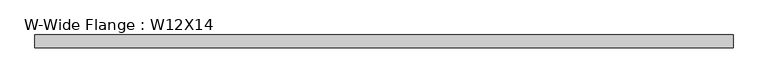
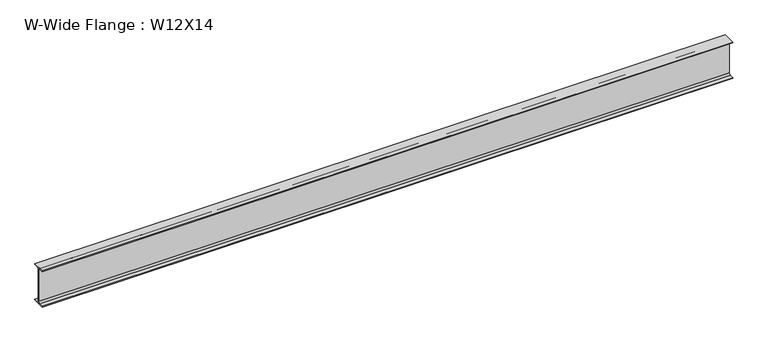
"""IFC4 building model written with IfcOpenShell, lengths in millimetres: beam geometry, W-Wide Flange : W12X14."""

from ifc_helpers import new_model, si_unit, point, frame, frame_2d, origin, place, context, project, spatial, polyline, circle_curve, trimmed, segment, composite_curve, outline, extrude, source, transform, mapped, element, save


def w_wide_flange_w12x14_09843c95(model_context):
    return source(origin(), model_context, "Body", "SweptSolid", [
        extrude(outline(composite_curve([segment(polyline([(50.419, -145.415), (50.419, -151.13), (-50.419, -151.13), (-50.419, -145.415), (-15.875, -145.415)]), True, "CONTINUOUS"), segment(trimmed(circle_curve(frame_2d((-15.875, -132.08)), 13.335), [point((-15.875, -145.415))], [point((-2.54, -132.08))], True, "CARTESIAN"), True, "CONTINUOUS"), segment(polyline([(-2.54, -132.08), (-2.54, 132.08)]), True, "CONTINUOUS"), segment(trimmed(circle_curve(frame_2d((-15.875, 132.08)), 13.335), [point((-2.54, 132.08))], [point((-15.875, 145.415))], True, "CARTESIAN"), True, "CONTINUOUS"), segment(polyline([(-15.875, 145.415), (-50.419, 145.415), (-50.419, 151.13), (50.419, 151.13), (50.419, 145.415), (15.875, 145.415)]), True, "CONTINUOUS"), segment(trimmed(circle_curve(frame_2d((15.875, 132.08)), 13.335), [point((15.875, 145.415))], [point((2.54, 132.08))], True, "CARTESIAN"), True, "CONTINUOUS"), segment(polyline([(2.54, 132.08), (2.54, -132.08)]), True, "CONTINUOUS"), segment(trimmed(circle_curve(frame_2d((15.875, -132.08)), 13.335), [point((2.54, -132.08))], [point((15.875, -145.415))], True, "CARTESIAN"), True, "CONTINUOUS"), segment(polyline([(15.875, -145.415), (50.419, -145.415)]), True, "CONTINUOUS")], self_intersect=False)), frame((-2743.327, 0.0, 0.0), z_axis=(1.0, 0.0, 0.0), x_axis=(0.0, 1.0, 0.0)), (0.0, 0.0, 1.0), 5474.335),
    ])


if __name__ == "__main__":
    model = new_model("IFC4")
    model_context = context("Model", 3, world=origin())
    ifc_project = project(units=[si_unit("LENGTHUNIT", "METRE", prefix="MILLI")], contexts=[model_context])
    site = spatial("IfcSite", under=ifc_project)
    building = spatial("IfcBuilding", under=site)
    placement = place(None, origin())
    w_wide_flange_w12x14_shape = w_wide_flange_w12x14_09843c95(model_context)
    element("IfcBeam", 1, ObjectType="W-Wide Flange : W12X14", at=placement, inside=building, context=model_context, shape_type="MappedRepresentation", body=[
        mapped(w_wide_flange_w12x14_shape, transform((0.0, 0.0, 0.0), x_axis=(1.0, 0.0, 0.0), y_axis=(0.0, 1.0, 0.0), z_axis=(0.0, 0.0, 1.0))),
    ])
    save(model, "model.ifc")

# Revit data of these elements
# Type "W-Wide Flange : W12X14"
#   Assembly Code = "B10"
#   W = 14
#   Length [instance default] = 5' - 0"
#   bf = 0' - 3.97"
#   d = 0' - 11.9"
#   k = 0' - 0 3/4"
#   k2 = 0' - 0.525"
#   tf = 0' - 0.225"
#   tw = 0' - 0.2"
#   A = 0.0288889 SF
#   Structural Material [instance default] = Steel ASTM A992
# Element 1 (IfcBeam, "W-Wide Flange : W12X14")
#   Materials on its faces: "Steel ASTM A992"
# Materials
#   "Steel ASTM A992": class "Metal", colour RGB 199 199 199, transparency 0, Description = "Structural steel 50ksi", Cost = 0
